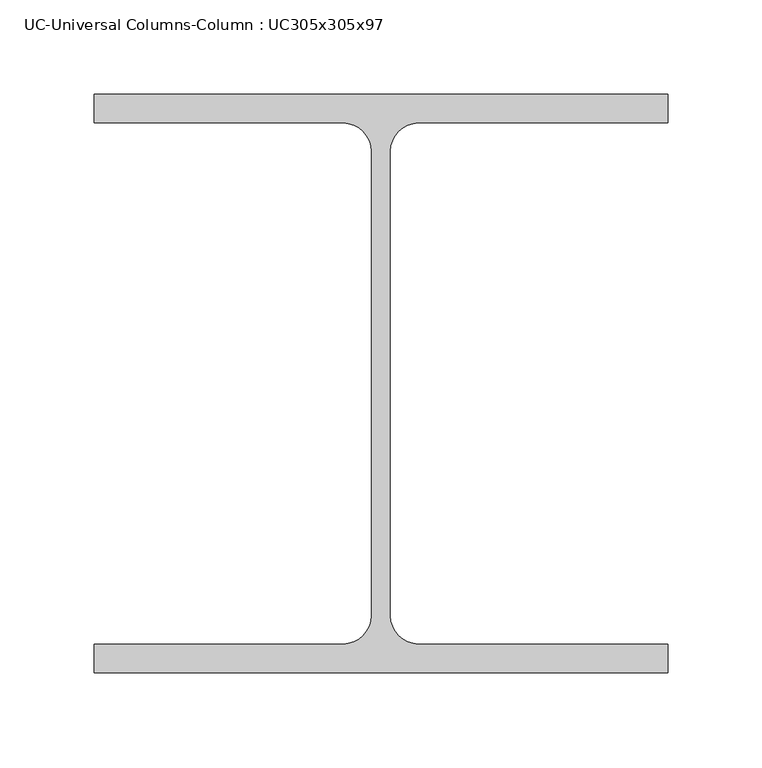
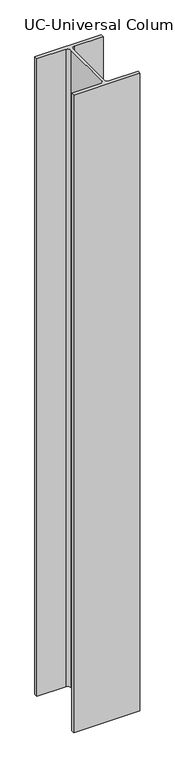
"""IFC4 building model written with IfcOpenShell, lengths in millimetres: column geometry, UC-Universal Columns-Column : UC305x305x97."""

import ifcopenshell
import ifcopenshell.guid

model = None  # the IFC model being written
_history = None  # IfcOwnerHistory: only IFC2X3 demands one
_inside = {}  # id of a spatial element -> (the spatial element, [elements in it])
_under = {}  # id of a project, library or spatial element -> (it, [spatial elements below it])
_declared = {}  # id of a project -> (the project, [libraries it declares])
_typed = {}  # id of a type object -> (the type object, [elements of that type])
_made_of = {}  # id of a material, layer set ... -> (it, [elements and type objects made of it])


def new_model(schema):
    """Start an empty IFC model of exactly this schema.

    Asked for "IFC4X3", IfcOpenShell would pick the latest addendum, in which some entities
    have other attributes; the version numbers below select the first issue.
    IFC2X3 requires an IfcOwnerHistory on every rooted entity: one is made here for all.
    """
    global model, _history
    if schema == "IFC4X3":
        model = ifcopenshell.file(schema_version=(4, 3, 0, 0))
    else:
        model = ifcopenshell.file(schema=schema)
    _inside.clear()
    _under.clear()
    _declared.clear()
    _typed.clear()
    _made_of.clear()
    _history = None
    if model.schema == "IFC2X3":
        org = make("IfcOrganization", Name="unknown")
        user = make(
            "IfcPersonAndOrganization",
            ThePerson=make("IfcPerson", FamilyName="unknown"),
            TheOrganization=org,
        )
        app = make(
            "IfcApplication",
            ApplicationDeveloper=org,
            Version="unknown",
            ApplicationFullName="unknown",
            ApplicationIdentifier="unknown",
        )
        _history = make(
            "IfcOwnerHistory",
            OwningUser=user,
            OwningApplication=app,
            ChangeAction="ADDED",
            CreationDate=0,
        )
    return model


def make(cls, **values):
    """One entity of the class cls with the attributes given. An attribute that is None is left unset."""
    return model.create_entity(
        cls, **{name: value for name, value in values.items() if value is not None}
    )


def rooted(cls, **values):
    """An entity with a GlobalId (a new one), such as an element, a storey or a relation."""
    return make(cls, GlobalId=ifcopenshell.guid.new(), OwnerHistory=_history, **values)


def si_unit(unit_type, name, prefix=None):
    """IfcSIUnit, for example si_unit("LENGTHUNIT", "METRE", prefix="MILLI")."""
    return make("IfcSIUnit", UnitType=unit_type, Prefix=prefix, Name=name)


def assignment(units):
    """IfcUnitAssignment: the units of a project."""
    return None if units is None else make("IfcUnitAssignment", Units=units)


def point(xyz):
    """IfcCartesianPoint."""
    return None if xyz is None else make("IfcCartesianPoint", Coordinates=xyz)


def direction(xyz):
    """IfcDirection."""
    return None if xyz is None else make("IfcDirection", DirectionRatios=xyz)


def frame(location, z_axis=None, x_axis=None):
    """IfcAxis2Placement3D, a coordinate frame: its origin and axes. An axis left out is left unset."""
    return make(
        "IfcAxis2Placement3D",
        Location=point(location),
        Axis=direction(z_axis),
        RefDirection=direction(x_axis),
    )


def frame_2d(location, x_axis=None):
    """IfcAxis2Placement2D, a coordinate frame in the plane: its origin and x axis."""
    return make(
        "IfcAxis2Placement2D", Location=point(location), RefDirection=direction(x_axis)
    )


def origin():
    """The frame at (0, 0, 0) with its axes left unset."""
    return frame((0.0, 0.0, 0.0))


def place(relative_to, where):
    """IfcLocalPlacement: puts the frame where relative to a parent placement (None: the world)."""
    return make(
        "IfcLocalPlacement", PlacementRelTo=relative_to, RelativePlacement=where
    )


def context(
    kind, dimensions, precision=None, world=None, true_north=None, identifier=None
):
    """IfcGeometricRepresentationContext, for example the 3D "Model" context."""
    return make(
        "IfcGeometricRepresentationContext",
        ContextIdentifier=identifier,
        ContextType=kind,
        CoordinateSpaceDimension=dimensions,
        Precision=precision,
        WorldCoordinateSystem=world,
        TrueNorth=true_north,
    )


def project(units=None, contexts=None):
    """IfcProject with its units and contexts."""
    return rooted(
        "IfcProject",
        Name="project",
        RepresentationContexts=contexts,
        UnitsInContext=assignment(units),
    )


def spatial(cls, under=None, at=None, **own):
    """A site, building, storey or space (cls), placed at a placement, below another one or the project."""
    s = rooted(cls, ObjectPlacement=at, **own)
    if under is not None:
        _under.setdefault(under.id(), (under, []))[1].append(s)
    return s


def polyline(points):
    """IfcPolyline through the points."""
    return make("IfcPolyline", Points=[point(p) for p in points])


def circle_curve(where, radius):
    """IfcCircle in the frame where."""
    return make("IfcCircle", Position=where, Radius=radius)


def trimmed(basis, trim1, trim2, sense, master):
    """IfcTrimmedCurve: the piece of a basis curve between two trims."""
    return make(
        "IfcTrimmedCurve",
        BasisCurve=basis,
        Trim1=trim1,
        Trim2=trim2,
        SenseAgreement=sense,
        MasterRepresentation=master,
    )


def segment(curve, same_sense, transition):
    """IfcCompositeCurveSegment."""
    return make(
        "IfcCompositeCurveSegment",
        Transition=transition,
        SameSense=same_sense,
        ParentCurve=curve,
    )


def composite_curve(segments, self_intersect=None):
    """IfcCompositeCurve: segments joined end to end."""
    return make("IfcCompositeCurve", Segments=segments, SelfIntersect=self_intersect)


def outline(outer, holes=None, kind="AREA"):
    """IfcArbitraryClosedProfileDef: a profile drawn as a closed curve; with holes, ...WithVoids."""
    if holes is None:
        return make("IfcArbitraryClosedProfileDef", ProfileType=kind, OuterCurve=outer)
    return make(
        "IfcArbitraryProfileDefWithVoids",
        ProfileType=kind,
        OuterCurve=outer,
        InnerCurves=holes,
    )


def extrude(swept, where, along, depth):
    """IfcExtrudedAreaSolid: the profile swept, set in the frame where, extruded along a direction by depth."""
    return make(
        "IfcExtrudedAreaSolid",
        SweptArea=swept,
        Position=where,
        ExtrudedDirection=direction(along),
        Depth=depth,
    )


def shape(context_of_items, identifier, shape_type, items):
    """IfcShapeRepresentation: the items that make up one representation, for example the "Body"."""
    return make(
        "IfcShapeRepresentation",
        ContextOfItems=context_of_items,
        RepresentationIdentifier=identifier,
        RepresentationType=shape_type,
        Items=items,
    )


def source(mapping_origin, context_of_items, identifier, shape_type, items):
    """IfcRepresentationMap: a shape defined once, which mapped items show again and again."""
    return make(
        "IfcRepresentationMap",
        MappingOrigin=mapping_origin,
        MappedRepresentation=shape(context_of_items, identifier, shape_type, items),
    )


def transform(
    local_origin,
    x_axis=None,
    y_axis=None,
    z_axis=None,
    scale=None,
    scale2=None,
    scale3=None,
    uniform=True,
):
    """IfcCartesianTransformationOperator3D, or its non-uniform kind. x_axis, y_axis, z_axis: its Axis1, 2, 3."""
    if uniform:
        return make(
            "IfcCartesianTransformationOperator3D",
            Axis1=direction(x_axis),
            Axis2=direction(y_axis),
            LocalOrigin=point(local_origin),
            Scale=scale,
            Axis3=direction(z_axis),
        )
    return make(
        "IfcCartesianTransformationOperator3DnonUniform",
        Axis1=direction(x_axis),
        Axis2=direction(y_axis),
        LocalOrigin=point(local_origin),
        Scale=scale,
        Axis3=direction(z_axis),
        Scale2=scale2,
        Scale3=scale3,
    )


def mapped(mapping_source, mapping_target):
    """IfcMappedItem: shows the shape of a source again, moved by a transform."""
    return make(
        "IfcMappedItem", MappingSource=mapping_source, MappingTarget=mapping_target
    )


def made_of(thing, what):
    """Note that an element or type object is made of a material, layer set ...; save() writes the relation."""
    if what is not None:
        _made_of.setdefault(what.id(), (what, []))[1].append(thing)
    return thing


def element(
    cls,
    number,
    at=None,
    inside=None,
    cuts=None,
    type_object=None,
    material=None,
    context=None,
    identifier="Body",
    shape_type=None,
    held_by="IfcProductDefinitionShape",
    body=None,
    shapes=None,
    **own,
):
    """One element of the class cls, such as IfcWall. Its Tag is "e" and its number.

    at: its placement. inside: the storey or other place that contains it. cuts: it is an
    opening in that element (IfcRelVoidsElement). A single representation is given by context,
    identifier, shape_type and body (its items); several are given by shapes. held_by: the class
    of the entity that holds the representations. save() writes the other relations.
    """
    e = rooted(cls, Tag="e%d" % number, ObjectPlacement=at, **own)
    if body is not None:
        shapes = [shape(context, identifier, shape_type, body)]
    if shapes is not None:
        e.Representation = make(held_by, Representations=shapes)
    if inside is not None:
        _inside.setdefault(inside.id(), (inside, []))[1].append(e)
    if cuts is not None:
        rooted(
            "IfcRelVoidsElement", RelatingBuildingElement=cuts, RelatedOpeningElement=e
        )
    if type_object is not None:
        _typed.setdefault(type_object.id(), (type_object, []))[1].append(e)
    return made_of(e, material)


def aggregate(whole, parts):
    """IfcRelAggregates: a whole, such as a stair, and the parts it consists of."""
    return rooted("IfcRelAggregates", RelatingObject=whole, RelatedObjects=parts)


def save(model, path):
    """Write the relations noted so far, then the file.

    IfcRelAggregates (storeys below a building ...), IfcRelContainedInSpatialStructure (elements
    in a storey), IfcRelDefinesByType, IfcRelAssociatesMaterial and IfcRelDeclares: one each for
    every whole, place, type object, material and project.
    """
    for whole, parts in _under.values():
        aggregate(whole, parts)
    for where, things in _inside.values():
        rooted(
            "IfcRelContainedInSpatialStructure",
            RelatedElements=things,
            RelatingStructure=where,
        )
    for kind, things in _typed.values():
        rooted("IfcRelDefinesByType", RelatedObjects=things, RelatingType=kind)
    for what, things in _made_of.values():
        rooted("IfcRelAssociatesMaterial", RelatedObjects=things, RelatingMaterial=what)
    for by, libraries in _declared.values():
        rooted("IfcRelDeclares", RelatingContext=by, RelatedDefinitions=libraries)
    model.write(path)


def uc_universal_columns_column_uc305x305x97_b067ee91(model_context):
    return source(origin(), model_context, "Body", "SweptSolid", [
        extrude(outline(composite_curve([segment(polyline([(152.65, 153.95), (152.65, 138.55), (20.15, 138.55)]), True, "CONTINUOUS"), segment(trimmed(circle_curve(frame_2d((20.15, 123.35)), 15.2), [point((20.15, 138.55))], [point((4.95, 123.35))], True, "CARTESIAN"), True, "CONTINUOUS"), segment(polyline([(4.95, 123.35), (4.95, -123.35)]), True, "CONTINUOUS"), segment(trimmed(circle_curve(frame_2d((20.15, -123.35)), 15.2), [point((4.95, -123.35))], [point((20.15, -138.55))], True, "CARTESIAN"), True, "CONTINUOUS"), segment(polyline([(20.15, -138.55), (152.65, -138.55), (152.65, -153.95), (-152.65, -153.95), (-152.65, -138.55), (-20.15, -138.55)]), True, "CONTINUOUS"), segment(trimmed(circle_curve(frame_2d((-20.15, -123.35)), 15.2), [point((-20.15, -138.55))], [point((-4.95, -123.35))], True, "CARTESIAN"), True, "CONTINUOUS"), segment(polyline([(-4.95, -123.35), (-4.95, 123.35)]), True, "CONTINUOUS"), segment(trimmed(circle_curve(frame_2d((-20.15, 123.35)), 15.2), [point((-4.95, 123.35))], [point((-20.15, 138.55))], True, "CARTESIAN"), True, "CONTINUOUS"), segment(polyline([(-20.15, 138.55), (-152.65, 138.55), (-152.65, 153.95), (152.65, 153.95)]), True, "CONTINUOUS")], self_intersect=False)), frame((0.0, 0.0, 2900.0), z_axis=(0.0, 0.0, 1.0), x_axis=(1.0, 0.0, 0.0)), (0.0, 0.0, 1.0), 3100.0),
    ])


if __name__ == "__main__":
    model = new_model("IFC4")
    model_context = context("Model", 3, world=origin())
    ifc_project = project(units=[si_unit("LENGTHUNIT", "METRE", prefix="MILLI")], contexts=[model_context])
    site = spatial("IfcSite", under=ifc_project)
    building = spatial("IfcBuilding", under=site)
    placement = place(None, origin())
    uc_universal_columns_column_uc305x305x97_shape = uc_universal_columns_column_uc305x305x97_b067ee91(model_context)
    element("IfcColumn", 1, ObjectType="UC-Universal Columns-Column : UC305x305x97", at=placement, inside=building, context=model_context, shape_type="MappedRepresentation", body=[
        mapped(uc_universal_columns_column_uc305x305x97_shape, transform((0.0, 0.0, 0.0), x_axis=(1.0, 0.0, 0.0), y_axis=(0.0, 1.0, 0.0), z_axis=(0.0, 0.0, 1.0))),
    ])
    save(model, "model.ifc")

# Revit data of these elements
# Type "UC-Universal Columns-Column : UC305x305x97"
#   Section Name Key = "UC305x305x97"
#   Cost = 5
#   Width = 30.53 cm
#   Web Thickness = 0.99 cm
#   Web Fillet = 1.52 cm
#   Warping Constant = 1560000.0 cm⁶
#   Torsional Moment of Inertia = 91.20 cm⁴
#   Section Area = 123.0 cm²
#   Plastic Modulus weak axis = 726.0 cm³
#   Plastic Modulus strong axis = 1592.0 cm³
#   Nominal Weight = 96.8996 kgf/m
#   Moment of Inertia weak axis = 7308.00 cm⁴
#   Moment of Inertia strong axis = 22249.00 cm⁴
#   Height = 30.79 cm
#   Flange Thickness = 1.54 cm
#   Elastic Modulus weak axis = 479.0 cm³
#   Elastic Modulus strong axis = 1445.0 cm³
#   Centroid Vertical = 15.395 cm
#   Centroid Horizontal = 15.265 cm
#   Bolt Spacing = 14.0 cm
#   Structural Material [instance default] = Metal - Steel 43-275
#   Type Comments = ""
#   Assembly Code = ""
# Element 1 (IfcColumn, "UC-Universal Columns-Column : UC305x305x97")
#   Materials on its faces: "Metal - Steel 43-275"
# Materials
#   "Metal - Steel 43-275": class "Metal", colour RGB 247 247 247, transparency 0, Cost = 0
